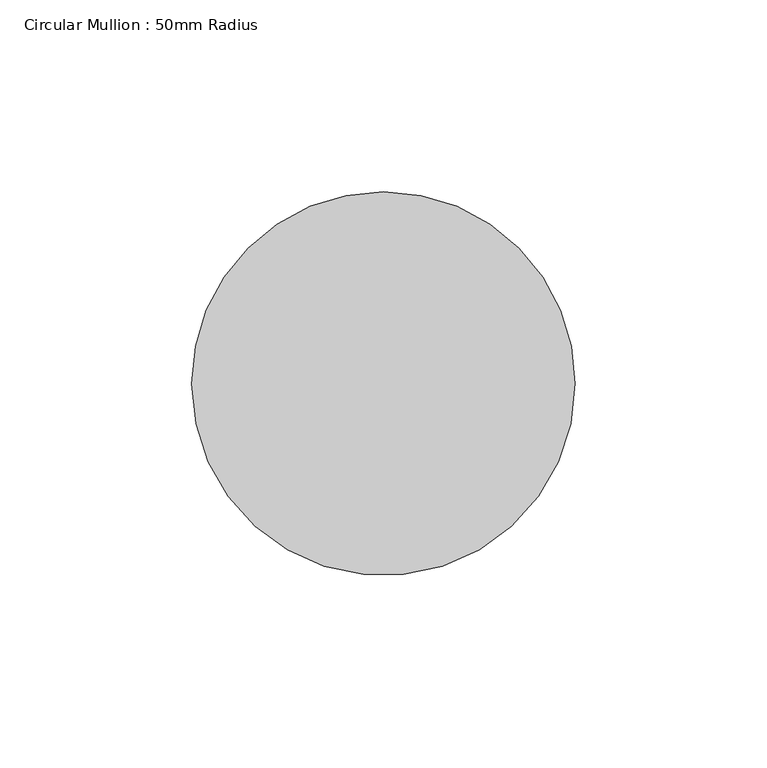
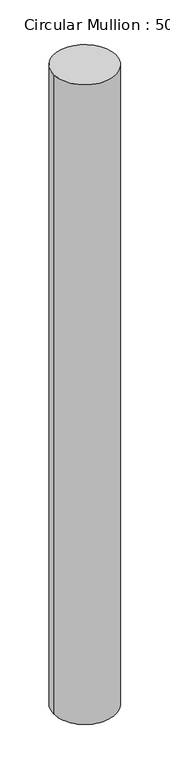
"""IFC4 building model written with IfcOpenShell, lengths in millimetres: member geometry, Circular Mullion : 50mm Radius."""

from ifc_helpers import new_model, si_unit, frame, origin, place, context, project, spatial, ellipse_curve, source, transform, mapped, element, save
from ifc_brep_helpers import plane_surface, cylinder_surface, advanced_brep


def circular_mullion_50mm_radius_052e3429(model_context):
    return source(origin(), model_context, "Body", "AdvancedBrep", [
        advanced_brep(
        [(-100.0, 0.0, 1.1470503), (0.0, 0.0, 0.0), (0.0, 0.0, -1082.8302473), (-100.0, 0.0, -1083.9383029)],
        [
            (0, 1, ellipse_curve(frame((-50.0, 0.0, 0.5735251), z_axis=(-0.011468484147785582, -0.014846057469093206, -0.9998240187397863), x_axis=(-0.6112241178838147, -0.7912352028102196, 0.018759838779243677)), 50.0088006, 50.0)),
            (1, 2),
            (2, 3, ellipse_curve(frame((-50.0, 0.0, -1083.3842751), z_axis=(-0.011078736807432496, -0.014341525977504956, 0.9998357776272003), x_axis=(0.6112313064645276, 0.7912445084934587, 0.01812230053308515)), 50.0082125, 50.0)),
            (3, 0),
            (1, 0, ellipse_curve(frame((-50.0, 0.0, 0.5735251), z_axis=(-0.011468484147785582, -0.014846057469093206, -0.9998240187397863), x_axis=(-0.6112241178838147, -0.7912352028102196, 0.018759838779243677)), 50.0088006, 50.0)),
            (3, 2, ellipse_curve(frame((-50.0, 0.0, -1083.3842751), z_axis=(-0.011078736807432496, -0.014341525977504956, 0.9998357776272003), x_axis=(0.6112313064645276, 0.7912445084934587, 0.01812230053308515)), 50.0082125, 50.0)),
        ],
        [
            cylinder_surface(frame((-50.0, 0.0, 0.0), z_axis=(0.0, 0.0, 1.0), x_axis=(1.0, 0.0, 0.0)), 50.0),
            plane_surface(frame((-241.2109384, 186.3339024, 0.0), z_axis=(0.011468484147785582, 0.014846057469093206, 0.9998240187397863), x_axis=(0.611224117883814, 0.79123520281022, -0.01875983877925467))),
            plane_surface(frame((-241.2109384, 186.3339024, -1082.8302473), z_axis=(0.011078736807432496, 0.014341525977504956, -0.9998357776272003), x_axis=(0.6112313064645274, 0.7912445084934588, 0.018122300533094826))),
        ],
        [
            (0, [[1, 2, 3, 4]]),
            (0, [[5, -4, 6, -2]]),
            (1, [[-1, -5]]),
            (2, [[-6, -3]]),
        ],
    ),
    ])


if __name__ == "__main__":
    model = new_model("IFC4")
    model_context = context("Model", 3, world=origin())
    ifc_project = project(units=[si_unit("LENGTHUNIT", "METRE", prefix="MILLI")], contexts=[model_context])
    site = spatial("IfcSite", under=ifc_project)
    building = spatial("IfcBuilding", under=site)
    placement = place(None, origin())
    circular_mullion_50mm_radius_shape = circular_mullion_50mm_radius_052e3429(model_context)
    element("IfcMember", 1, ObjectType="Circular Mullion : 50mm Radius", at=placement, inside=building, context=model_context, shape_type="MappedRepresentation", body=[
        mapped(circular_mullion_50mm_radius_shape, transform((0.0, 0.0, 0.0), x_axis=(1.0, 0.0, 0.0), y_axis=(0.0, 1.0, 0.0), z_axis=(0.0, 0.0, 1.0))),
    ])
    save(model, "model.ifc")

# Revit data of these elements
# Type "Circular Mullion : 50mm Radius"
#   built-in parameter 1007350 = 0.164042 (stored number, unit not read)
# Element 1 (IfcMember, "Circular Mullion : 50mm Radius")
#   Materials on its faces: "Aluminium"
# Materials
#   "Aluminium": class "Metal", colour RGB 247 247 247, transparency 0, Description = "Aluminium 6061", Cost = 0
